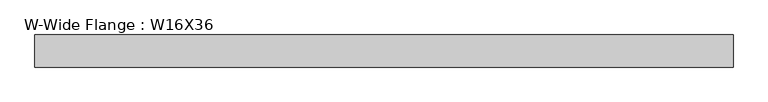
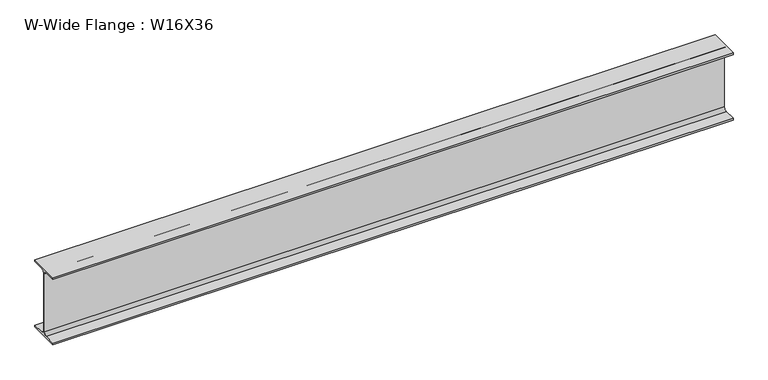
"""IFC4 building model written with IfcOpenShell, lengths in millimetres: beam geometry, W-Wide Flange : W16X36."""

from ifc_helpers import new_model, si_unit, point, frame, frame_2d, origin, place, context, project, spatial, polyline, circle_curve, trimmed, segment, composite_curve, outline, extrude, source, transform, mapped, element, save


def w_wide_flange_w16x36_590c5b68(model_context):
    return source(origin(), model_context, "Body", "SweptSolid", [
        extrude(outline(composite_curve([segment(polyline([(88.773, -191.008), (88.773, -201.93), (-88.773, -201.93), (-88.773, -191.008), (-21.3995, -191.008)]), True, "CONTINUOUS"), segment(trimmed(circle_curve(frame_2d((-21.3995, -173.355)), 17.653), [point((-21.3995, -191.008))], [point((-3.7465, -173.355))], True, "CARTESIAN"), True, "CONTINUOUS"), segment(polyline([(-3.7465, -173.355), (-3.7465, 173.355)]), True, "CONTINUOUS"), segment(trimmed(circle_curve(frame_2d((-21.3995, 173.355)), 17.653), [point((-3.7465, 173.355))], [point((-21.3995, 191.008))], True, "CARTESIAN"), True, "CONTINUOUS"), segment(polyline([(-21.3995, 191.008), (-88.773, 191.008), (-88.773, 201.93), (88.773, 201.93), (88.773, 191.008), (21.3995, 191.008)]), True, "CONTINUOUS"), segment(trimmed(circle_curve(frame_2d((21.3995, 173.355)), 17.653), [point((21.3995, 191.008))], [point((3.7465, 173.355))], True, "CARTESIAN"), True, "CONTINUOUS"), segment(polyline([(3.7465, 173.355), (3.7465, -173.355)]), True, "CONTINUOUS"), segment(trimmed(circle_curve(frame_2d((21.3995, -173.355)), 17.653), [point((3.7465, -173.355))], [point((21.3995, -191.008))], True, "CARTESIAN"), True, "CONTINUOUS"), segment(polyline([(21.3995, -191.008), (88.773, -191.008)]), True, "CONTINUOUS")], self_intersect=False)), frame((-1892.3, 0.0, 0.0), z_axis=(1.0, 0.0, 0.0), x_axis=(0.0, 1.0, 0.0)), (0.0, 0.0, 1.0), 3860.7999994),
    ])


if __name__ == "__main__":
    model = new_model("IFC4")
    model_context = context("Model", 3, world=origin())
    ifc_project = project(units=[si_unit("LENGTHUNIT", "METRE", prefix="MILLI")], contexts=[model_context])
    site = spatial("IfcSite", under=ifc_project)
    building = spatial("IfcBuilding", under=site)
    placement = place(None, origin())
    w_wide_flange_w16x36_shape = w_wide_flange_w16x36_590c5b68(model_context)
    element("IfcBeam", 1, ObjectType="W-Wide Flange : W16X36", at=placement, inside=building, context=model_context, shape_type="MappedRepresentation", body=[
        mapped(w_wide_flange_w16x36_shape, transform((0.0, 0.0, 0.0), x_axis=(1.0, 0.0, 0.0), y_axis=(0.0, 1.0, 0.0), z_axis=(0.0, 0.0, 1.0))),
    ])
    save(model, "model.ifc")

# Revit data of these elements
# Type "W-Wide Flange : W16X36"
#   Assembly Code = "B10"
#   W = 36
#   Length [instance default] = 5' - 0"
#   bf = 0' - 6.99"
#   d = 1' - 3.9"
#   k = 0' - 1 1/8"
#   k2 = 0' - 0.695"
#   tf = 0' - 0.43"
#   tw = 0' - 0.295"
#   A = 0.0736111 SF
#   Structural Material [instance default] = Steel ASTM A992
# Element 1 (IfcBeam, "W-Wide Flange : W16X36")
#   Materials on its faces: "Steel ASTM A992"
# Materials
#   "Steel ASTM A992": class "Metal", colour RGB 199 199 199, transparency 0, Description = "Structural steel 50ksi", Cost = 0
